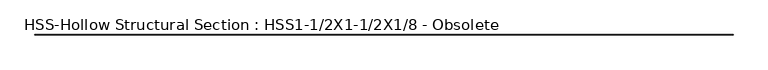
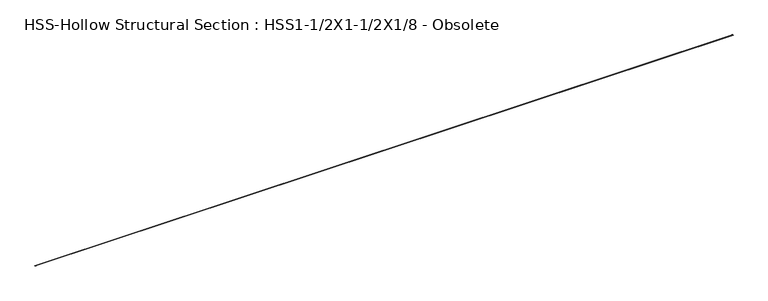
"""IFC4 building model written with IfcOpenShell, lengths in millimetres: beam geometry, HSS-Hollow Structural Section : HSS1-1/2X1-1/2X1/8 - Obsolete."""

from ifc_helpers import new_model, si_unit, point, frame, frame_2d, origin, place, context, project, spatial, polyline, circle_curve, trimmed, segment, composite_curve, outline, extrude, source, transform, mapped, element, save


def hss_hollow_structural_section_hss1_1_2x1_1_2x1_8_obsolete_11a1fb5f(model_context):
    return source(origin(), model_context, "Body", "SweptSolid", [
        extrude(outline(composite_curve([segment(polyline([(19.05, 13.1572), (19.05, -13.1572)]), True, "CONTINUOUS"), segment(trimmed(circle_curve(frame_2d((13.1572, -13.1572)), 5.8928), [point((19.05, -13.1572))], [point((13.1572, -19.05))], False, "CARTESIAN"), True, "CONTINUOUS"), segment(polyline([(13.1572, -19.05), (-13.1572, -19.05)]), True, "CONTINUOUS"), segment(trimmed(circle_curve(frame_2d((-13.1572, -13.1572)), 5.8928), [point((-13.1572, -19.05))], [point((-19.05, -13.1572))], False, "CARTESIAN"), True, "CONTINUOUS"), segment(polyline([(-19.05, -13.1572), (-19.05, 13.1572)]), True, "CONTINUOUS"), segment(trimmed(circle_curve(frame_2d((-13.1572, 13.1572)), 5.8928), [point((-19.05, 13.1572))], [point((-13.1572, 19.05))], False, "CARTESIAN"), True, "CONTINUOUS"), segment(polyline([(-13.1572, 19.05), (13.1572, 19.05)]), True, "CONTINUOUS"), segment(trimmed(circle_curve(frame_2d((13.1572, 13.1572)), 5.8928), [point((13.1572, 19.05))], [point((19.05, 13.1572))], False, "CARTESIAN"), True, "CONTINUOUS")], self_intersect=False), holes=[composite_curve([segment(trimmed(circle_curve(frame_2d((-13.1572, 13.1572)), 2.9464), [point((-13.1572, 16.1036))], [point((-16.1036, 13.1572))], True, "CARTESIAN"), True, "CONTINUOUS"), segment(polyline([(-16.1036, 13.1572), (-16.1036, -13.1572)]), True, "CONTINUOUS"), segment(trimmed(circle_curve(frame_2d((-13.1572, -13.1572)), 2.9464), [point((-16.1036, -13.1572))], [point((-13.1572, -16.1036))], True, "CARTESIAN"), True, "CONTINUOUS"), segment(polyline([(-13.1572, -16.1036), (13.1572, -16.1036)]), True, "CONTINUOUS"), segment(trimmed(circle_curve(frame_2d((13.1572, -13.1572)), 2.9464), [point((13.1572, -16.1036))], [point((16.1036, -13.1572))], True, "CARTESIAN"), True, "CONTINUOUS"), segment(polyline([(16.1036, -13.1572), (16.1036, 13.1572)]), True, "CONTINUOUS"), segment(trimmed(circle_curve(frame_2d((13.1572, 13.1572)), 2.9464), [point((16.1036, 13.1572))], [point((13.1572, 16.1036))], True, "CARTESIAN"), True, "CONTINUOUS"), segment(polyline([(13.1572, 16.1036), (-13.1572, 16.1036)]), True, "CONTINUOUS")], self_intersect=False)]), frame((-44523.0377, 0.0, 0.0), z_axis=(1.0, 0.0, 0.0), x_axis=(0.0, 1.0, 0.0)), (0.0, 0.0, 1.0), 89046.0754),
    ])


if __name__ == "__main__":
    model = new_model("IFC4")
    model_context = context("Model", 3, world=origin())
    ifc_project = project(units=[si_unit("LENGTHUNIT", "METRE", prefix="MILLI")], contexts=[model_context])
    site = spatial("IfcSite", under=ifc_project)
    building = spatial("IfcBuilding", under=site)
    placement = place(None, origin())
    hss_hollow_structural_section_hss1_1_2x1_1_2x1_8_obsolete_shape = hss_hollow_structural_section_hss1_1_2x1_1_2x1_8_obsolete_11a1fb5f(model_context)
    element("IfcBeam", 1, ObjectType="HSS-Hollow Structural Section : HSS1-1/2X1-1/2X1/8 - Obsolete", at=placement, inside=building, context=model_context, shape_type="MappedRepresentation", body=[
        mapped(hss_hollow_structural_section_hss1_1_2x1_1_2x1_8_obsolete_shape, transform((0.0, 0.0, 0.0), x_axis=(1.0, 0.0, 0.0), y_axis=(0.0, 1.0, 0.0), z_axis=(0.0, 0.0, 1.0))),
    ])
    save(model, "model.ifc")

# Revit data of these elements
# Type "HSS-Hollow Structural Section : HSS1-1/2X1-1/2X1/8 - Obsolete"
#   Assembly Code = "B10"
#   Shape = "Square"
#   W = 2.19
#   Ht = 0' - 1 1/2"
#   Length [instance default] = 5' - 0"
#   b = 0' - 1 1/2"
#   kr = 0' - 0.232"
#   t = 0' - 0.116"
#   A = 0.00423611 SF
#   Structural Material [instance default] = 1 1/2" X 1 1/2" SPLIT-SEAM SQUARE TUBING (~24" CANTILEVER FROM C.L. OF GLULAM)
# Element 1 (IfcBeam, "HSS-Hollow Structural Section : HSS1-1/2X1-1/2X1/8 - Obsolete")
#   Materials on its faces: "1 1/2\" X 1 1/2\" SPLIT-SEAM SQUARE TUBING (~24\" CANTILEVER FROM C.L. OF GLULAM)"
# Materials
#   "1 1/2\" X 1 1/2\" SPLIT-SEAM SQUARE TUBING (~24\" CANTILEVER FROM C.L. OF GLULAM)": class "Metal", colour RGB 199 199 199, transparency 0, Description = "Carbon steel", Cost = 0
